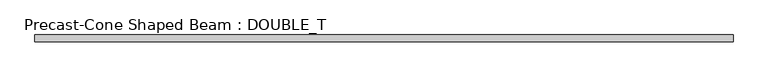
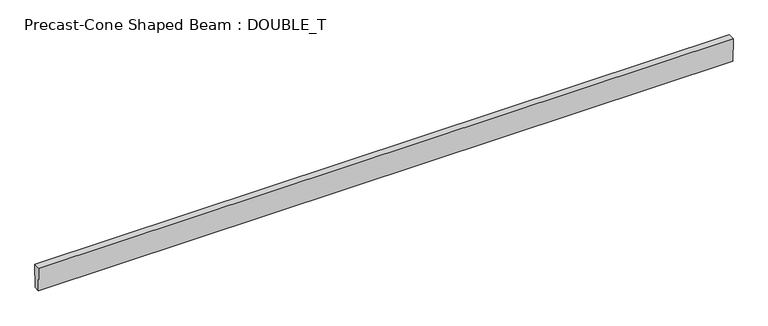
"""IFC4 building model written with IfcOpenShell, lengths in millimetres: beam geometry, Precast-Cone Shaped Beam : DOUBLE_T."""

from ifc_helpers import new_model, si_unit, frame, origin, place, context, project, spatial, polyline, outline, extrude, source, transform, mapped, element, save


def precast_cone_shaped_beam_double_t_099a914b(model_context):
    return source(origin(), model_context, "Body", "SweptSolid", [
        extrude(outline(polyline([(50.8, -228.6), (-50.8, -228.6), (-63.5, 228.6), (63.5, 228.6), (50.8, -228.6)])), frame((-6574.63125, 0.0, 0.0), z_axis=(1.0, 0.0, 0.0), x_axis=(0.0, 1.0, 0.0)), (0.0, 0.0, 1.0), 13208.0),
    ])


if __name__ == "__main__":
    model = new_model("IFC4")
    model_context = context("Model", 3, world=origin())
    ifc_project = project(units=[si_unit("LENGTHUNIT", "METRE", prefix="MILLI")], contexts=[model_context])
    site = spatial("IfcSite", under=ifc_project)
    building = spatial("IfcBuilding", under=site)
    placement = place(None, origin())
    precast_cone_shaped_beam_double_t_shape = precast_cone_shaped_beam_double_t_099a914b(model_context)
    element("IfcBeam", 1, ObjectType="Precast-Cone Shaped Beam : DOUBLE_T", at=placement, inside=building, context=model_context, shape_type="MappedRepresentation", body=[
        mapped(precast_cone_shaped_beam_double_t_shape, transform((0.0, 0.0, 0.0), x_axis=(1.0, 0.0, 0.0), y_axis=(0.0, 1.0, 0.0), z_axis=(0.0, 0.0, 1.0))),
    ])
    save(model, "model.ifc")

# Revit data of these elements
# Type "Precast-Cone Shaped Beam : DOUBLE_T"
#   Top Width = 0' - 5"
#   Tie Rod Weight [instance default] = 30
#   Tie Rod W [instance default] = 0.0660938 kip
#   Single Rebar Weight [instance default] = 50
#   Single Rebar W [instance default] = 0.110156 kip
#   Rebar Grids Weight [instance default] = 100
#   Rebar Grids W [instance default] = 0.220313 kip
#   Depth = 1' - 6"
#   Bottom Width = 0' - 4"
#   Length [instance default] = 5' - 0"
#   Structural Material [instance default] = Concrete, Precast
#   Assembly Code = ""
# Element 1 (IfcBeam, "Precast-Cone Shaped Beam : DOUBLE_T")
#   Length = 42' - 9 11/16"
#   Structural Material = Concrete - Precast Concrete - Normal Weight Concrete - 5 ksi
#   Materials on its faces: "Concrete - Precast Concrete - Normal Weight Concrete - 5 ksi"
# Materials
#   "Concrete, Precast": class "Concrete", colour RGB 198 187 187, transparency 0, Description = "Precast concrete", Cost = 0
#   "Concrete - Precast Concrete - Normal Weight Concrete - 5 ksi": class "Concrete", colour RGB 198 187 187, transparency 0, Cost = 0
